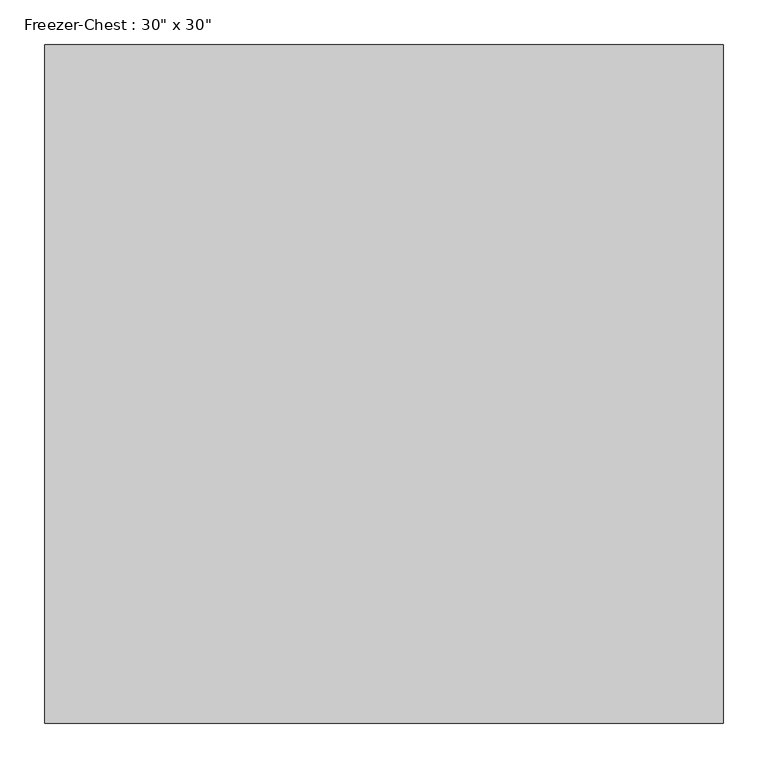
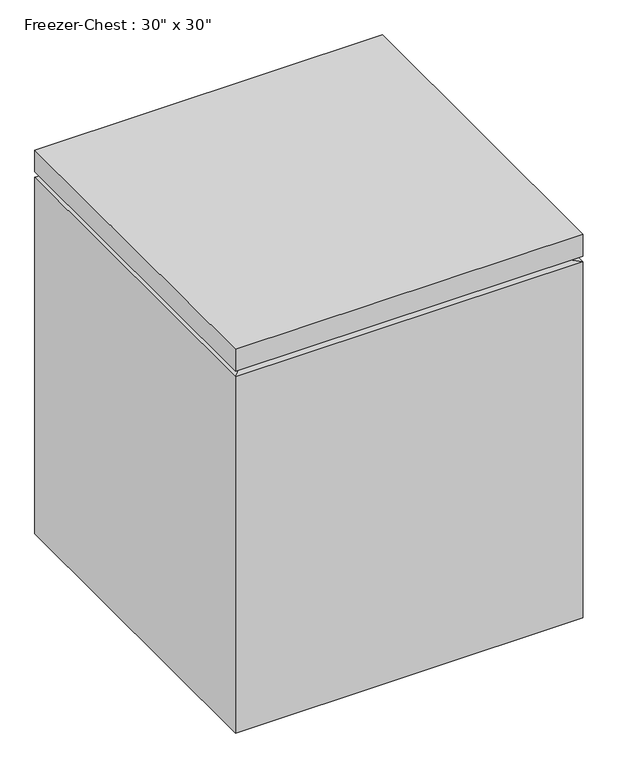
"""IFC4 building model written with IfcOpenShell, lengths in millimetres: proxy geometry."""

from ifc_helpers import new_model, si_unit, frame, origin, place, context, project, spatial, polyline, outline, extrude, faceted_brep, source, transform, mapped, element, save


def proxy_cdf8c592(model_context):
    return source(origin(), model_context, "Body", "SolidModel", [
        faceted_brep([(381.0, 381.0, 889.0), (-381.0, 381.0, 889.0), (-381.0, -381.0, 889.0), (381.0, -381.0, 889.0), (381.0, 381.0, 0.0), (381.0, -381.0, 0.0), (-381.0, -381.0, 0.0), (-381.0, 381.0, 0.0), (381.0, 381.0, 838.2), (361.95, 381.0, 838.2), (361.95, 381.0, 825.5), (381.0, 381.0, 825.5), (-381.0, 381.0, 825.5), (-361.95, 381.0, 825.5), (-361.95, 381.0, 838.2), (-381.0, 381.0, 838.2), (-381.0, -381.0, 838.2), (-381.0, -381.0, 825.5), (381.0, -381.0, 838.2), (381.0, -381.0, 825.5), (361.95, -361.95, 838.2), (361.95, -361.95, 825.5), (-361.95, -361.95, 838.2), (-361.95, -361.95, 825.5)], [[[0, 1, 2, 3]], [[4, 5, 6, 7]], [[1, 0, 8, 9, 10, 11, 4, 7, 12, 13, 14, 15]], [[2, 1, 15, 16]], [[7, 6, 17, 12]], [[3, 2, 16, 18]], [[6, 5, 19, 17]], [[0, 3, 18, 8]], [[5, 4, 11, 19]], [[18, 20, 9, 8]], [[10, 21, 19, 11]], [[9, 20, 21, 10]], [[20, 18, 16, 22]], [[19, 21, 23, 17]], [[21, 20, 22, 23]], [[22, 16, 15, 14]], [[17, 23, 13, 12]], [[23, 22, 14, 13]]]),
        extrude(outline(polyline([(-355.6, 879.475), (-355.6, 847.8538878), (-361.95, 847.8538878), (-361.95, 873.2538878), (-374.65, 873.2538878), (-374.65, 879.475), (-355.6, 879.475)])), frame((-54.3302756, 0.0, 0.0), z_axis=(1.0, 0.0, 0.0), x_axis=(0.0, 1.0, 0.0)), (0.0, 0.0, 1.0), 101.6),
    ])


if __name__ == "__main__":
    model = new_model("IFC4")
    model_context = context("Model", 3, world=origin())
    ifc_project = project(units=[si_unit("LENGTHUNIT", "METRE", prefix="MILLI")], contexts=[model_context])
    site = spatial("IfcSite", under=ifc_project)
    building = spatial("IfcBuilding", under=site)
    placement = place(None, origin())
    proxy_shape = proxy_cdf8c592(model_context)
    element("IfcBuildingElementProxy", 1, Name="Freezer-Chest : 30\" x 30\"", ObjectType="Freezer-Chest : 30\" x 30\"", at=placement, inside=building, context=model_context, shape_type="MappedRepresentation", body=[
        mapped(proxy_shape, transform((0.0, 0.0, 0.0), x_axis=(1.0, 0.0, 0.0), y_axis=(0.0, 1.0, 0.0), z_axis=(0.0, 0.0, 1.0))),
    ])
    save(model, "model.ifc")

# Revit data of these elements
# Type "Freezer-Chest : 30\" x 30\""
#   COBie.Type.CreatedBy = "design@eagle.com"
#   COBie.Type.CreatedOn = "2016-10-27T05:31:12"
#   COBie.Type.Name = "Freezer-Chest_30\" x 30\""
#   COBie.Type.Category = "E1090400"
#   COBie.Type.Description = "Freezer-Chest_30\" x 30\""
#   COBie.Type.Manufacturer = ""
#   COBie.Type.ModelNumber = ""
#   Assembly Code = "E1090400"
#   COBie.Type.ReplacementCost = 0
#   Depth = 2' - 6"
#   Height = 2' - 11"
#   Width = 2' - 6"
#   COBie.Type = yes
#   Material = Metal - Paint Finish - Ivory,Glossy
# Element 1 (IfcBuildingElementProxy, "Freezer-Chest : 30\" x 30\"")
#   Materials on its faces: "Metal - Paint Finish - Ivory,Glossy"
# Materials
#   "Metal - Paint Finish - Ivory,Glossy": class "Metal", colour RGB 247 247 239, transparency 0
